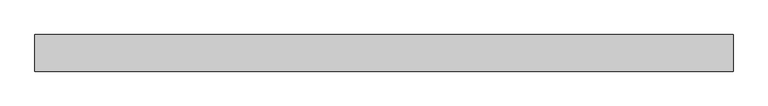
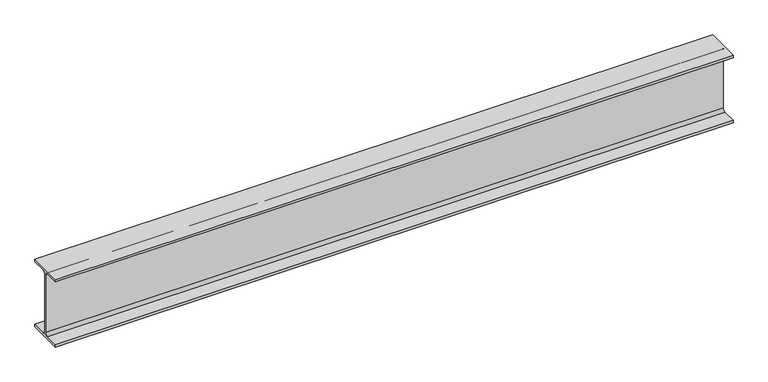
"""IFC4 building model written with IfcOpenShell, lengths in millimetres: beam geometry, 0912_Steel Framing_H-KSD3502 : H_SB_ASB_H-400x200x8x13."""

from ifc_helpers import new_model, si_unit, point, frame, frame_2d, origin, place, context, project, spatial, polyline, circle_curve, trimmed, segment, composite_curve, outline, extrude, source, transform, mapped, element, save


def beam_3114dbc3(model_context):
    return source(origin(), model_context, "Body", "SweptSolid", [
        extrude(outline(composite_curve([segment(polyline([(100.0, -187.0), (100.0, -200.0), (-100.0, -200.0), (-100.0, -187.0), (-20.0, -187.0)]), True, "CONTINUOUS"), segment(trimmed(circle_curve(frame_2d((-20.0, -171.0)), 16.0), [point((-20.0, -187.0))], [point((-4.0, -171.0))], True, "CARTESIAN"), True, "CONTINUOUS"), segment(polyline([(-4.0, -171.0), (-4.0, 171.0)]), True, "CONTINUOUS"), segment(trimmed(circle_curve(frame_2d((-20.0, 171.0)), 16.0), [point((-4.0, 171.0))], [point((-20.0, 187.0))], True, "CARTESIAN"), True, "CONTINUOUS"), segment(polyline([(-20.0, 187.0), (-100.0, 187.0), (-100.0, 200.0), (100.0, 200.0), (100.0, 187.0), (20.0, 187.0)]), True, "CONTINUOUS"), segment(trimmed(circle_curve(frame_2d((20.0, 171.0)), 16.0), [point((20.0, 187.0))], [point((4.0, 171.0))], True, "CARTESIAN"), True, "CONTINUOUS"), segment(polyline([(4.0, 171.0), (4.0, -171.0)]), True, "CONTINUOUS"), segment(trimmed(circle_curve(frame_2d((20.0, -171.0)), 16.0), [point((4.0, -171.0))], [point((20.0, -187.0))], True, "CARTESIAN"), True, "CONTINUOUS"), segment(polyline([(20.0, -187.0), (100.0, -187.0)]), True, "CONTINUOUS")], self_intersect=False)), frame((-1904.8, 0.0, 0.0), z_axis=(1.0, 0.0, 0.0), x_axis=(0.0, 1.0, 0.0)), (0.0, 0.0, 1.0), 3809.6),
    ])


if __name__ == "__main__":
    model = new_model("IFC4")
    model_context = context("Model", 3, world=origin())
    ifc_project = project(units=[si_unit("LENGTHUNIT", "METRE", prefix="MILLI")], contexts=[model_context])
    site = spatial("IfcSite", under=ifc_project)
    building = spatial("IfcBuilding", under=site)
    placement = place(None, origin())
    beam_shape = beam_3114dbc3(model_context)
    element("IfcBeam", 1, ObjectType="0912_Steel Framing_H-KSD3502 : H_SB_ASB_H-400x200x8x13", at=placement, inside=building, context=model_context, shape_type="MappedRepresentation", body=[
        mapped(beam_shape, transform((0.0, 0.0, 0.0), x_axis=(1.0, 0.0, 0.0), y_axis=(0.0, 1.0, 0.0), z_axis=(0.0, 0.0, 1.0))),
    ])
    save(model, "model.ifc")

# Revit data of these elements
# Type "0912_Steel Framing_H-KSD3502 : H_SB_ASB_H-400x200x8x13"
#   H_WM Code_1 = "S01AA002-00001 | Main Steel Structure Fabrication Work | Shelter/Building | Medium Steel - Standard (90KG/M>Weight≥30KG/M) | Material: (   )"
#   H_WM Code_2 = "S03AA028-00001 | Main Steel Structure Erection Work | Shelter/Building | Medium Steel (90KG/M>Weight≥30KG/M) | Material: (   )"
#   H_WM Code_3 = "S01AA010-00001 | Main Steel Structure Fabrication Work | Shelter/Building | Steel Painting/Coating | for Non-Fireproofed Steel Surface, Surface Preparation, Primer, Second & Final Coat | Material: (   )"
#   H_Q'ty Cal Type Tag = "SB-Q2"
#   Width = 20.0 cm
#   Web Thickness = 0.8 cm
#   Web Fillet = 1.6 cm
#   Warping Constant = 649000.0 cm⁶
#   W = 0
#   Torsional Moment of Inertia = 35.8981 cm⁴
#   Section Area = 84.12 cm²
#   Plastic Modulus weak axis = 268.0 cm³
#   Plastic Modulus strong axis = 1330.0 cm³
#   Perimeter = 1.56 m²/m
#   Nominal Weight = 66.00 kgf/m
#   Moment of Inertia weak axis = 1740.00 cm⁴
#   Moment of Inertia strong axis = 23700.00 cm⁴
#   Height = 40.0 cm
#   Flange Thickness = 1.3 cm
#   Elastic Modulus weak axis = 174.0 cm³
#   Elastic Modulus strong axis = 1190.0 cm³
#   Centroid Vertical = 20.0 cm
#   Centroid Horizontal = 10.0 cm
#   Ix = 237000000
#   Length [instance default] = 1.5240 m
#   Zx = 1330000
#   b = 0.2000 m
#   h = 0.4000 m
#   r = 0.0160 m
#   s = 0.0080 m
#   t = 0.0130 m
#   A = 0.008412 m²
#   Structural Material [instance default] = Steel, 45-345
#   Assembly Code = ""
# Element 1 (IfcBeam, "0912_Steel Framing_H-KSD3502 : H_SB_ASB_H-400x200x8x13")
#   Structural Material = none
# Materials
#   "Steel, 45-345": class "Metal", colour RGB 189 187 185, transparency 0, Description = "Steel 345 MPa", Cost = 0
